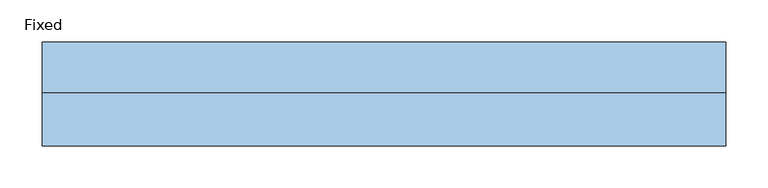
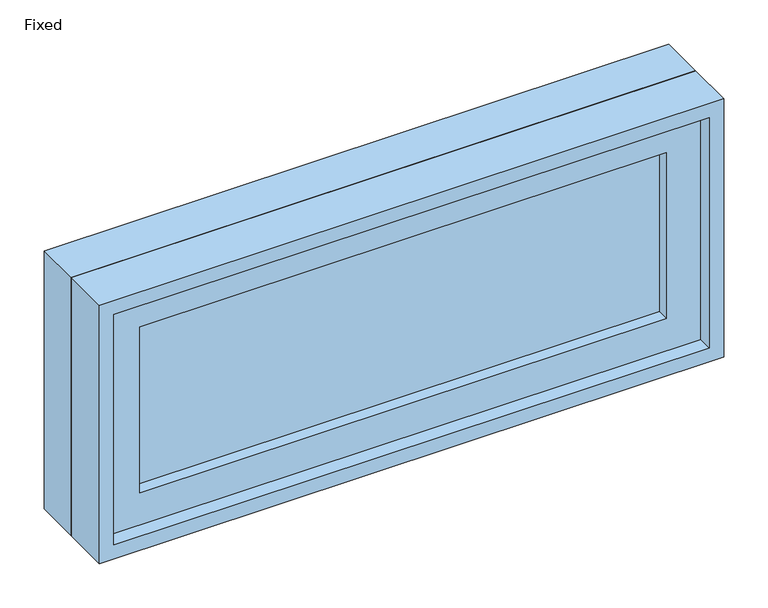
"""IFC4 building model written with IfcOpenShell, lengths in millimetres: window geometry, Fixed."""

from ifc_helpers import new_model, si_unit, frame, origin, place, context, project, spatial, polyline, outline, extrude, source, transform, mapped, element, save


def fixed_17397640(model_context):
    return source(origin(), model_context, "Body", "SweptSolid", [
        extrude(outline(polyline([(304.8, -14.2875), (304.8, -26.9875), (-381.0, -26.9875), (-381.0, -14.2875), (304.8, -14.2875)])), frame((0.0, 0.0, 24447.5), z_axis=(0.0, 0.0, 1.0), x_axis=(1.0, 0.0, 0.0)), (0.0, 0.0, 1.0), 228.6),
        extrude(outline(polyline([(24720.55, -425.45), (24403.05, -425.45), (24403.05, 349.25), (24720.55, 349.25), (24720.55, -425.45)]), holes=[polyline([(24676.1, -381.0), (24676.1, 304.8), (24447.5, 304.8), (24447.5, -381.0), (24676.1, -381.0)])]), frame((0.0, -42.8625, 0.0), z_axis=(0.0, 1.0, 0.0), x_axis=(0.0, 0.0, 1.0)), (0.0, 0.0, 1.0), 44.45),
        extrude(outline(polyline([(24739.6, -444.5), (24384.0, -444.5), (24384.0, 368.3), (24739.6, 368.3), (24739.6, -444.5)]), holes=[polyline([(24707.85, -412.75), (24707.85, 336.55), (24415.75, 336.55), (24415.75, -412.75), (24707.85, -412.75)])]), frame((0.0, 1.5875, 0.0), z_axis=(0.0, 1.0, 0.0), x_axis=(0.0, 0.0, 1.0)), (0.0, 0.0, 1.0), 60.325),
        extrude(outline(polyline([(24739.6, 368.3), (24739.6, -444.5), (24384.0, -444.5), (24384.0, 368.3), (24739.6, 368.3)]), holes=[polyline([(24720.55, 349.25), (24403.05, 349.25), (24403.05, -425.45), (24720.55, -425.45), (24720.55, 349.25)])]), frame((0.0, -61.9125, 0.0), z_axis=(0.0, 1.0, 0.0), x_axis=(0.0, 0.0, 1.0)), (0.0, 0.0, 1.0), 63.5),
    ])


if __name__ == "__main__":
    model = new_model("IFC4")
    model_context = context("Model", 3, world=origin())
    ifc_project = project(units=[si_unit("LENGTHUNIT", "METRE", prefix="MILLI")], contexts=[model_context])
    site = spatial("IfcSite", under=ifc_project)
    building = spatial("IfcBuilding", under=site)
    placement = place(None, origin())
    fixed_shape = fixed_17397640(model_context)
    element("IfcWindow", 1, ObjectType="Fixed : 14\" x 32\"  Screen", at=placement, inside=building, context=model_context, shape_type="MappedRepresentation", body=[
        mapped(fixed_shape, transform((0.0, 0.0, 0.0), x_axis=(1.0, 0.0, 0.0), y_axis=(0.0, 1.0, 0.0), z_axis=(0.0, 0.0, 1.0))),
    ])
    save(model, "model.ifc")

# Revit data of these elements
# Type "Fixed : 14\" x 32\"  Screen"
#   Type Mark = "72"
#   COBie.Type.CreatedBy = "doug.wood@us.ibm.com"
#   COBie.Type.CreatedOn = "2016-04-14T02:07:26"
#   COBie.Type.Name = "Windows_Fixed_14\" x 32\"  Screen_72"
#   COBie.Type.Category = "23-30 20 17 11 : Fixed Windows"
#   COBie.Type.Description = "Fixed_14\" x 32\"  Screen"
#   COBie.Type.Manufacturer = ""
#   COBie.Type.ModelNumber = ""
#   Construction Type Id = "GSP4R"
#   Assembly Code = "B2020100"
#   Analytic Construction = "1/8 in Pilkington single glazing"
#   COBie.Type.ReplacementCost = 0
#   Visual Light Transmittance = 0.9
#   Solar Heat Gain Coefficient = 0.78
#   Heat Transfer Coefficient (U) = 3.6886 W/(m²·K)
#   Height = 1' - 2"
#   Default Sill Height = 80' - 0"
#   Width = 2' - 8"
#   Window Inset = 0' - 0 3/4"
#   COBie.Type = no
#   Glass Pane Material = Screen
#   Sash Material = Sash - White
#   Wall Closure = (empty or 0)
# Element 1 (IfcWindow, "Fixed : 14\" x 32\"  Screen")
#   Materials on its faces: "Sash - White", "Screen"
# Materials
#   "Screen": class "Metal", colour RGB 120 120 120, transparency 0, Description = "Screen", Cost = 0
#   "Sash - White": class "Wood", colour RGB 255 255 255, transparency 0, Cost = 0
